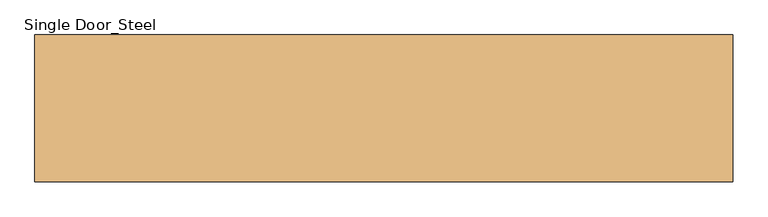
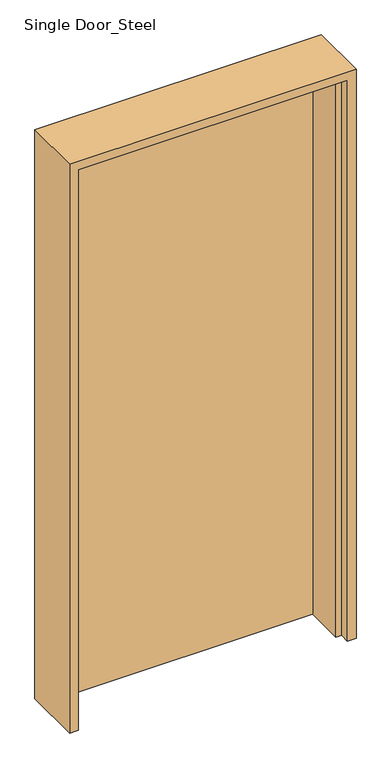
"""IFC4 building model written with IfcOpenShell, lengths in millimetres: door geometry, Single Door_Steel : H_DR_AR_B12_Single Door_Steel_W1000xH2100."""

from ifc_helpers import new_model, si_unit, origin, origin_with_axes, place, context, project, spatial, polyline, outline, extrude, faceted_brep, source, transform, mapped, element, save


def single_door_steel_6218e75e(model_context):
    return source(origin(), model_context, "Body", "SolidModel", [
        extrude(outline(polyline([(470.0, 105.0), (470.0, 70.0), (-470.0, 70.0), (-470.0, 105.0), (470.0, 105.0)])), origin_with_axes(), (0.0, 0.0, 1.0), 2070.0),
        faceted_brep([(470.0, 105.0, 0.0), (500.0, 105.0, 0.0), (500.0, -105.0, 0.0), (470.0, -105.0, 0.0), (470.0, -70.0, 0.0), (450.0, -70.0, 0.0), (450.0, 70.0, 0.0), (470.0, 70.0, 0.0), (470.0, 105.0, 2070.0), (-470.0, 105.0, 2070.0), (-470.0, 105.0, 0.0), (-500.0, 105.0, 0.0), (-500.0, 105.0, 2100.0), (500.0, 105.0, 2100.0), (500.0, -105.0, 2100.0), (-500.0, -105.0, 2100.0), (-500.0, -105.0, 0.0), (-470.0, -105.0, 0.0), (-470.0, -105.0, 2070.0), (470.0, -105.0, 2070.0), (470.0, -70.0, 2070.0), (-470.0, -70.0, 2070.0), (-470.0, -70.0, 0.0), (-450.0, -70.0, 0.0), (-450.0, -70.0, 2050.0), (450.0, -70.0, 2050.0), (450.0, 70.0, 2050.0), (-450.0, 70.0, 2050.0), (-450.0, 70.0, 0.0), (-470.0, 70.0, 0.0), (-470.0, 70.0, 2070.0), (470.0, 70.0, 2070.0)], [[[0, 1, 2, 3, 4, 5, 6, 7]], [[1, 0, 8, 9, 10, 11, 12, 13]], [[2, 1, 13, 14]], [[3, 2, 14, 15, 16, 17, 18, 19]], [[4, 3, 19, 20]], [[5, 4, 20, 21, 22, 23, 24, 25]], [[6, 5, 25, 26]], [[7, 6, 26, 27, 28, 29, 30, 31]], [[0, 7, 31, 8]], [[9, 30, 29, 10]], [[10, 29, 28, 23, 22, 17, 16, 11]], [[15, 12, 11, 16]], [[21, 18, 17, 22]], [[27, 24, 23, 28]], [[14, 13, 12, 15]], [[20, 19, 18, 21]], [[26, 25, 24, 27]], [[8, 31, 30, 9]]]),
    ])


if __name__ == "__main__":
    model = new_model("IFC4")
    model_context = context("Model", 3, world=origin())
    ifc_project = project(units=[si_unit("LENGTHUNIT", "METRE", prefix="MILLI")], contexts=[model_context])
    site = spatial("IfcSite", under=ifc_project)
    building = spatial("IfcBuilding", under=site)
    placement = place(None, origin())
    single_door_steel_shape = single_door_steel_6218e75e(model_context)
    element("IfcDoor", 1, ObjectType="Single Door_Steel : H_DR_AR_B12_Single Door_Steel_W1000xH2100", at=placement, inside=building, context=model_context, shape_type="MappedRepresentation", body=[
        mapped(single_door_steel_shape, transform((0.0, 0.0, 0.0), x_axis=(1.0, 0.0, 0.0), y_axis=(0.0, 1.0, 0.0), z_axis=(0.0, 0.0, 1.0))),
    ])
    save(model, "model.ifc")

# Revit data of these elements
# Type "Single Door_Steel : H_DR_AR_B12_Single Door_Steel_W1000xH2100"
#   Type Mark = "SD"
#   Analytic Construction = "<None>"
#   프레임 투영 외부. = 25 mm
#   프레임 투영 내부. = 25 mm
#   프레임 폭 = 75 mm
#   Height = 2100 mm
#   Width = 1000 mm
#   Define Thermal Properties by = 1
#   문 패널 = none
#   문 프레임 = none
#   Function = (empty or 0)
#   Wall Closure = (empty or 0)
